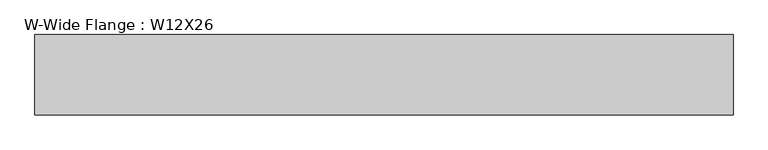
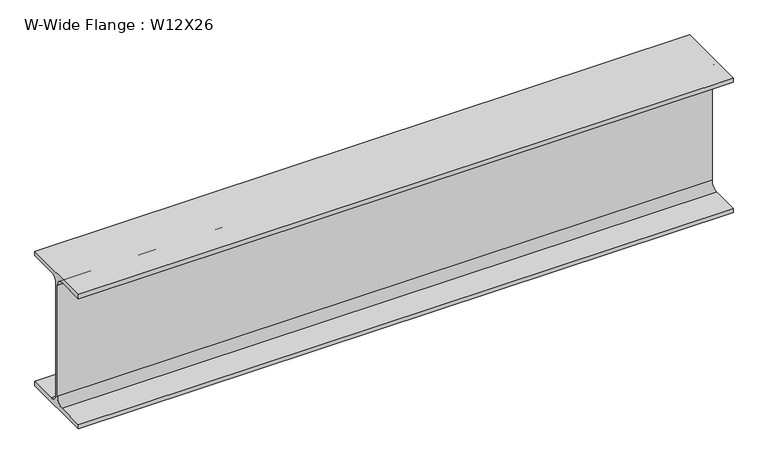
"""IFC4 building model written with IfcOpenShell, lengths in millimetres: beam geometry, W-Wide Flange : W12X26."""

import ifcopenshell
import ifcopenshell.guid

model = None  # the IFC model being written
_history = None  # IfcOwnerHistory: only IFC2X3 demands one
_inside = {}  # id of a spatial element -> (the spatial element, [elements in it])
_under = {}  # id of a project, library or spatial element -> (it, [spatial elements below it])
_declared = {}  # id of a project -> (the project, [libraries it declares])
_typed = {}  # id of a type object -> (the type object, [elements of that type])
_made_of = {}  # id of a material, layer set ... -> (it, [elements and type objects made of it])


def new_model(schema):
    """Start an empty IFC model of exactly this schema.

    Asked for "IFC4X3", IfcOpenShell would pick the latest addendum, in which some entities
    have other attributes; the version numbers below select the first issue.
    IFC2X3 requires an IfcOwnerHistory on every rooted entity: one is made here for all.
    """
    global model, _history
    if schema == "IFC4X3":
        model = ifcopenshell.file(schema_version=(4, 3, 0, 0))
    else:
        model = ifcopenshell.file(schema=schema)
    _inside.clear()
    _under.clear()
    _declared.clear()
    _typed.clear()
    _made_of.clear()
    _history = None
    if model.schema == "IFC2X3":
        org = make("IfcOrganization", Name="unknown")
        user = make(
            "IfcPersonAndOrganization",
            ThePerson=make("IfcPerson", FamilyName="unknown"),
            TheOrganization=org,
        )
        app = make(
            "IfcApplication",
            ApplicationDeveloper=org,
            Version="unknown",
            ApplicationFullName="unknown",
            ApplicationIdentifier="unknown",
        )
        _history = make(
            "IfcOwnerHistory",
            OwningUser=user,
            OwningApplication=app,
            ChangeAction="ADDED",
            CreationDate=0,
        )
    return model


def make(cls, **values):
    """One entity of the class cls with the attributes given. An attribute that is None is left unset."""
    return model.create_entity(
        cls, **{name: value for name, value in values.items() if value is not None}
    )


def rooted(cls, **values):
    """An entity with a GlobalId (a new one), such as an element, a storey or a relation."""
    return make(cls, GlobalId=ifcopenshell.guid.new(), OwnerHistory=_history, **values)


def si_unit(unit_type, name, prefix=None):
    """IfcSIUnit, for example si_unit("LENGTHUNIT", "METRE", prefix="MILLI")."""
    return make("IfcSIUnit", UnitType=unit_type, Prefix=prefix, Name=name)


def assignment(units):
    """IfcUnitAssignment: the units of a project."""
    return None if units is None else make("IfcUnitAssignment", Units=units)


def point(xyz):
    """IfcCartesianPoint."""
    return None if xyz is None else make("IfcCartesianPoint", Coordinates=xyz)


def direction(xyz):
    """IfcDirection."""
    return None if xyz is None else make("IfcDirection", DirectionRatios=xyz)


def frame(location, z_axis=None, x_axis=None):
    """IfcAxis2Placement3D, a coordinate frame: its origin and axes. An axis left out is left unset."""
    return make(
        "IfcAxis2Placement3D",
        Location=point(location),
        Axis=direction(z_axis),
        RefDirection=direction(x_axis),
    )


def frame_2d(location, x_axis=None):
    """IfcAxis2Placement2D, a coordinate frame in the plane: its origin and x axis."""
    return make(
        "IfcAxis2Placement2D", Location=point(location), RefDirection=direction(x_axis)
    )


def origin():
    """The frame at (0, 0, 0) with its axes left unset."""
    return frame((0.0, 0.0, 0.0))


def place(relative_to, where):
    """IfcLocalPlacement: puts the frame where relative to a parent placement (None: the world)."""
    return make(
        "IfcLocalPlacement", PlacementRelTo=relative_to, RelativePlacement=where
    )


def context(
    kind, dimensions, precision=None, world=None, true_north=None, identifier=None
):
    """IfcGeometricRepresentationContext, for example the 3D "Model" context."""
    return make(
        "IfcGeometricRepresentationContext",
        ContextIdentifier=identifier,
        ContextType=kind,
        CoordinateSpaceDimension=dimensions,
        Precision=precision,
        WorldCoordinateSystem=world,
        TrueNorth=true_north,
    )


def project(units=None, contexts=None):
    """IfcProject with its units and contexts."""
    return rooted(
        "IfcProject",
        Name="project",
        RepresentationContexts=contexts,
        UnitsInContext=assignment(units),
    )


def spatial(cls, under=None, at=None, **own):
    """A site, building, storey or space (cls), placed at a placement, below another one or the project."""
    s = rooted(cls, ObjectPlacement=at, **own)
    if under is not None:
        _under.setdefault(under.id(), (under, []))[1].append(s)
    return s


def polyline(points):
    """IfcPolyline through the points."""
    return make("IfcPolyline", Points=[point(p) for p in points])


def circle_curve(where, radius):
    """IfcCircle in the frame where."""
    return make("IfcCircle", Position=where, Radius=radius)


def trimmed(basis, trim1, trim2, sense, master):
    """IfcTrimmedCurve: the piece of a basis curve between two trims."""
    return make(
        "IfcTrimmedCurve",
        BasisCurve=basis,
        Trim1=trim1,
        Trim2=trim2,
        SenseAgreement=sense,
        MasterRepresentation=master,
    )


def segment(curve, same_sense, transition):
    """IfcCompositeCurveSegment."""
    return make(
        "IfcCompositeCurveSegment",
        Transition=transition,
        SameSense=same_sense,
        ParentCurve=curve,
    )


def composite_curve(segments, self_intersect=None):
    """IfcCompositeCurve: segments joined end to end."""
    return make("IfcCompositeCurve", Segments=segments, SelfIntersect=self_intersect)


def outline(outer, holes=None, kind="AREA"):
    """IfcArbitraryClosedProfileDef: a profile drawn as a closed curve; with holes, ...WithVoids."""
    if holes is None:
        return make("IfcArbitraryClosedProfileDef", ProfileType=kind, OuterCurve=outer)
    return make(
        "IfcArbitraryProfileDefWithVoids",
        ProfileType=kind,
        OuterCurve=outer,
        InnerCurves=holes,
    )


def extrude(swept, where, along, depth):
    """IfcExtrudedAreaSolid: the profile swept, set in the frame where, extruded along a direction by depth."""
    return make(
        "IfcExtrudedAreaSolid",
        SweptArea=swept,
        Position=where,
        ExtrudedDirection=direction(along),
        Depth=depth,
    )


def shape(context_of_items, identifier, shape_type, items):
    """IfcShapeRepresentation: the items that make up one representation, for example the "Body"."""
    return make(
        "IfcShapeRepresentation",
        ContextOfItems=context_of_items,
        RepresentationIdentifier=identifier,
        RepresentationType=shape_type,
        Items=items,
    )


def source(mapping_origin, context_of_items, identifier, shape_type, items):
    """IfcRepresentationMap: a shape defined once, which mapped items show again and again."""
    return make(
        "IfcRepresentationMap",
        MappingOrigin=mapping_origin,
        MappedRepresentation=shape(context_of_items, identifier, shape_type, items),
    )


def transform(
    local_origin,
    x_axis=None,
    y_axis=None,
    z_axis=None,
    scale=None,
    scale2=None,
    scale3=None,
    uniform=True,
):
    """IfcCartesianTransformationOperator3D, or its non-uniform kind. x_axis, y_axis, z_axis: its Axis1, 2, 3."""
    if uniform:
        return make(
            "IfcCartesianTransformationOperator3D",
            Axis1=direction(x_axis),
            Axis2=direction(y_axis),
            LocalOrigin=point(local_origin),
            Scale=scale,
            Axis3=direction(z_axis),
        )
    return make(
        "IfcCartesianTransformationOperator3DnonUniform",
        Axis1=direction(x_axis),
        Axis2=direction(y_axis),
        LocalOrigin=point(local_origin),
        Scale=scale,
        Axis3=direction(z_axis),
        Scale2=scale2,
        Scale3=scale3,
    )


def mapped(mapping_source, mapping_target):
    """IfcMappedItem: shows the shape of a source again, moved by a transform."""
    return make(
        "IfcMappedItem", MappingSource=mapping_source, MappingTarget=mapping_target
    )


def made_of(thing, what):
    """Note that an element or type object is made of a material, layer set ...; save() writes the relation."""
    if what is not None:
        _made_of.setdefault(what.id(), (what, []))[1].append(thing)
    return thing


def element(
    cls,
    number,
    at=None,
    inside=None,
    cuts=None,
    type_object=None,
    material=None,
    context=None,
    identifier="Body",
    shape_type=None,
    held_by="IfcProductDefinitionShape",
    body=None,
    shapes=None,
    **own,
):
    """One element of the class cls, such as IfcWall. Its Tag is "e" and its number.

    at: its placement. inside: the storey or other place that contains it. cuts: it is an
    opening in that element (IfcRelVoidsElement). A single representation is given by context,
    identifier, shape_type and body (its items); several are given by shapes. held_by: the class
    of the entity that holds the representations. save() writes the other relations.
    """
    e = rooted(cls, Tag="e%d" % number, ObjectPlacement=at, **own)
    if body is not None:
        shapes = [shape(context, identifier, shape_type, body)]
    if shapes is not None:
        e.Representation = make(held_by, Representations=shapes)
    if inside is not None:
        _inside.setdefault(inside.id(), (inside, []))[1].append(e)
    if cuts is not None:
        rooted(
            "IfcRelVoidsElement", RelatingBuildingElement=cuts, RelatedOpeningElement=e
        )
    if type_object is not None:
        _typed.setdefault(type_object.id(), (type_object, []))[1].append(e)
    return made_of(e, material)


def aggregate(whole, parts):
    """IfcRelAggregates: a whole, such as a stair, and the parts it consists of."""
    return rooted("IfcRelAggregates", RelatingObject=whole, RelatedObjects=parts)


def save(model, path):
    """Write the relations noted so far, then the file.

    IfcRelAggregates (storeys below a building ...), IfcRelContainedInSpatialStructure (elements
    in a storey), IfcRelDefinesByType, IfcRelAssociatesMaterial and IfcRelDeclares: one each for
    every whole, place, type object, material and project.
    """
    for whole, parts in _under.values():
        aggregate(whole, parts)
    for where, things in _inside.values():
        rooted(
            "IfcRelContainedInSpatialStructure",
            RelatedElements=things,
            RelatingStructure=where,
        )
    for kind, things in _typed.values():
        rooted("IfcRelDefinesByType", RelatedObjects=things, RelatingType=kind)
    for what, things in _made_of.values():
        rooted("IfcRelAssociatesMaterial", RelatedObjects=things, RelatingMaterial=what)
    for by, libraries in _declared.values():
        rooted("IfcRelDeclares", RelatingContext=by, RelatedDefinitions=libraries)
    model.write(path)


def w_wide_flange_w12x26_5cfc586e(model_context):
    return source(origin(), model_context, "Body", "SweptSolid", [
        extrude(outline(composite_curve([segment(polyline([(-82.4011719, -145.5539063), (-20.2902344, -145.5539063)]), True, "CONTINUOUS"), segment(trimmed(circle_curve(frame_2d((-20.2902344, -128.190625)), 17.3632812), [point((-20.2902344, -145.5539063))], [point((-2.9269531, -128.190625))], True, "CARTESIAN"), True, "CONTINUOUS"), segment(polyline([(-2.9269531, -128.190625), (-2.9269531, 128.190625)]), True, "CONTINUOUS"), segment(trimmed(circle_curve(frame_2d((-20.2902344, 128.190625)), 17.3632812), [point((-2.9269531, 128.190625))], [point((-20.2902344, 145.5539062))], True, "CARTESIAN"), True, "CONTINUOUS"), segment(polyline([(-20.2902344, 145.5539062), (-82.4011719, 145.5539062), (-82.4011719, 155.178125), (82.4011719, 155.178125), (82.4011719, 145.5539062), (20.2902344, 145.5539062)]), True, "CONTINUOUS"), segment(trimmed(circle_curve(frame_2d((20.2902344, 128.190625)), 17.3632812), [point((20.2902344, 145.5539062))], [point((2.9269531, 128.190625))], True, "CARTESIAN"), True, "CONTINUOUS"), segment(polyline([(2.9269531, 128.190625), (2.9269531, -128.190625)]), True, "CONTINUOUS"), segment(trimmed(circle_curve(frame_2d((20.2902344, -128.190625)), 17.3632812), [point((2.9269531, -128.190625))], [point((20.2902344, -145.5539063))], True, "CARTESIAN"), True, "CONTINUOUS"), segment(polyline([(20.2902344, -145.5539063), (82.4011719, -145.5539063), (82.4011719, -155.178125), (-82.4011719, -155.178125), (-82.4011719, -145.5539063)]), True, "CONTINUOUS")], self_intersect=False)), frame((-666.8988281, 0.0, 0.0), z_axis=(1.0, 0.0, 0.0), x_axis=(0.0, 1.0, 0.0)), (0.0, 0.0, 1.0), 1428.8988281),
    ])


if __name__ == "__main__":
    model = new_model("IFC4")
    model_context = context("Model", 3, world=origin())
    ifc_project = project(units=[si_unit("LENGTHUNIT", "METRE", prefix="MILLI")], contexts=[model_context])
    site = spatial("IfcSite", under=ifc_project)
    building = spatial("IfcBuilding", under=site)
    placement = place(None, origin())
    w_wide_flange_w12x26_shape = w_wide_flange_w12x26_5cfc586e(model_context)
    element("IfcBeam", 1, ObjectType="W-Wide Flange : W12X26", at=placement, inside=building, context=model_context, shape_type="MappedRepresentation", body=[
        mapped(w_wide_flange_w12x26_shape, transform((0.0, 0.0, 0.0), x_axis=(1.0, 0.0, 0.0), y_axis=(0.0, 1.0, 0.0), z_axis=(0.0, 0.0, 1.0))),
    ])
    save(model, "model.ifc")

# Revit data of these elements
# Type "W-Wide Flange : W12X26"
#   Assembly Code = "B10"
#   W = 26
#   Start Extension Calculation [instance default] = 10' - 0"
#   Start Extension [instance default] = -0' - 0 1/2"
#   End Extension Calculation [instance default] = 10' - 0"
#   End Extension [instance default] = -0' - 0 1/2"
#   Length [instance default] = 5' - 0"
#   bf = 0' - 6 125/256"
#   d = 1' - 0 7/32"
#   k = 0' - 1 1/16"
#   k2 = 0' - 0 175/256"
#   tf = 0' - 0 97/256"
#   tw = 0' - 0 59/256"
#   A = 0.05 SF
#   Beam Material [instance default] = Metal - Steel - ASTM A992
# Element 1 (IfcBeam, "W-Wide Flange : W12X26")
#   Materials on its faces: "Metal - Steel - ASTM A992"
# Materials
#   "Metal - Steel - ASTM A992": class "Metal", colour RGB 128 0 0, transparency 0
